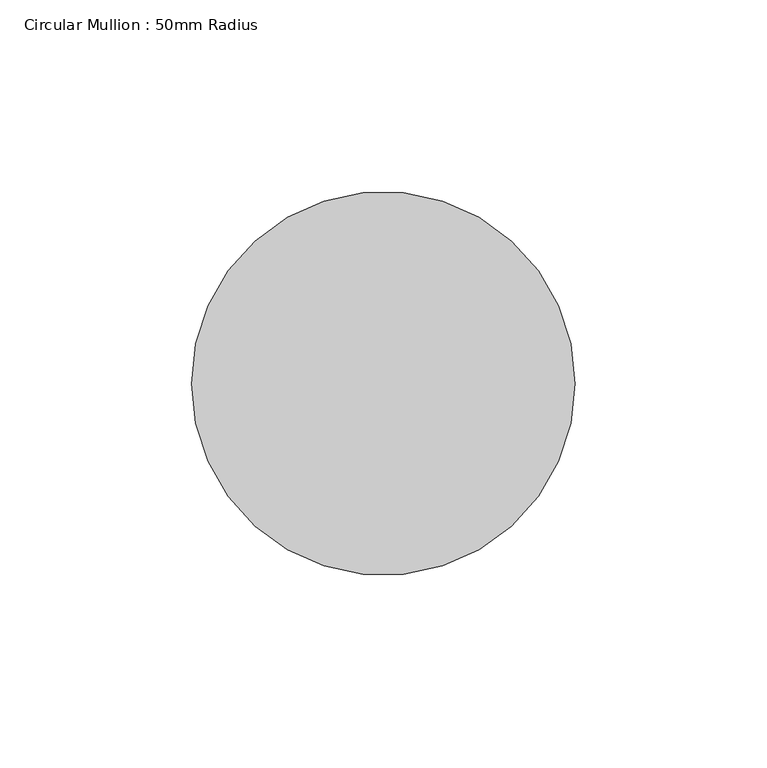
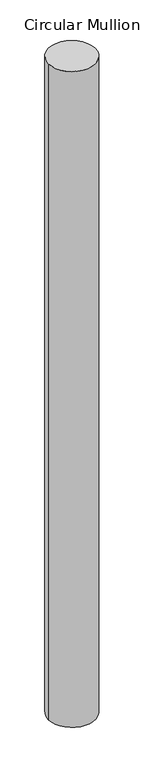
"""IFC4 building model written with IfcOpenShell, lengths in millimetres: member geometry, Circular Mullion : 50mm Radius."""

from ifc_helpers import new_model, si_unit, point, frame, origin, origin_2d, place, context, project, spatial, circle_curve, trimmed, segment, composite_curve, outline, extrude, source, transform, mapped, element, save


def circular_mullion_50mm_radius_1042f9b4(model_context):
    return source(origin(), model_context, "Body", "SweptSolid", [
        extrude(outline(composite_curve([segment(trimmed(circle_curve(origin_2d(), 50.0), [point((50.0, 0.0))], [point((-50.0, 0.0))], False, "CARTESIAN"), True, "CONTINUOUS"), segment(trimmed(circle_curve(origin_2d(), 50.0), [point((-50.0, 0.0))], [point((50.0, 0.0))], False, "CARTESIAN"), True, "CONTINUOUS")], self_intersect=False)), frame((0.0, 0.0, -1480.2509426), z_axis=(0.0, 0.0, 1.0), x_axis=(1.0, 0.0, 0.0)), (0.0, 0.0, 1.0), 1480.2509426),
    ])


if __name__ == "__main__":
    model = new_model("IFC4")
    model_context = context("Model", 3, world=origin())
    ifc_project = project(units=[si_unit("LENGTHUNIT", "METRE", prefix="MILLI")], contexts=[model_context])
    site = spatial("IfcSite", under=ifc_project)
    building = spatial("IfcBuilding", under=site)
    placement = place(None, origin())
    circular_mullion_50mm_radius_shape = circular_mullion_50mm_radius_1042f9b4(model_context)
    element("IfcMember", 1, ObjectType="Circular Mullion : 50mm Radius", at=placement, inside=building, context=model_context, shape_type="MappedRepresentation", body=[
        mapped(circular_mullion_50mm_radius_shape, transform((0.0, 0.0, 0.0), x_axis=(1.0, 0.0, 0.0), y_axis=(0.0, 1.0, 0.0), z_axis=(0.0, 0.0, 1.0))),
    ])
    save(model, "model.ifc")

# Revit data of these elements
# Type "Circular Mullion : 50mm Radius"
#   built-in parameter 1007350 = 0.164042 (stored number, unit not read)
# Element 1 (IfcMember, "Circular Mullion : 50mm Radius")
#   Materials on its faces: "Aluminium"
# Materials
#   "Aluminium": class "Metal", colour RGB 247 247 247, transparency 0, Description = "Aluminium 6061", Cost = 0
